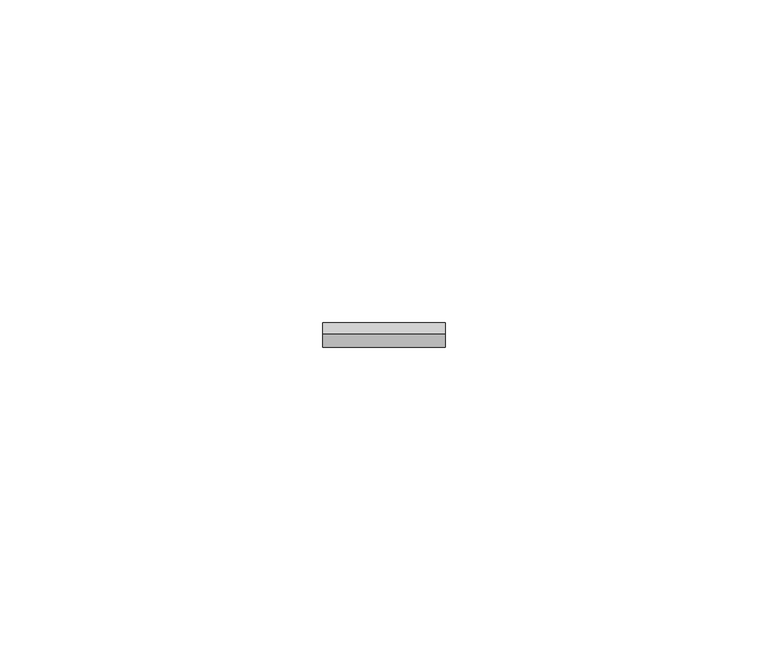
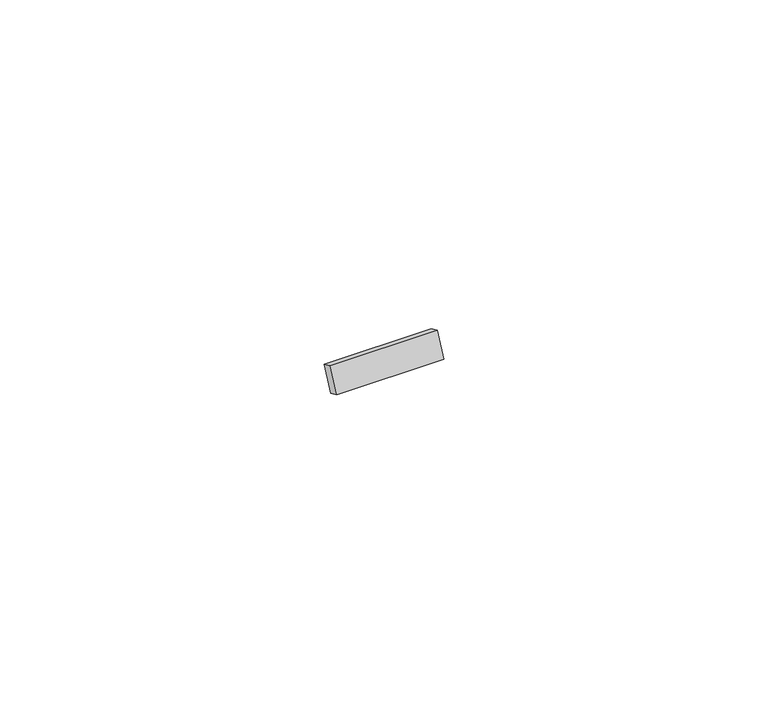
"""IFC4 building model written with IfcOpenShell, lengths in millimetres: furniture geometry, MOLDURA TELA1 : MOLDURA TELA."""

from ifc_helpers import new_model, si_unit, frame, origin, place, context, project, spatial, polyline, outline, extrude, source, transform, mapped, element, save


def furniture_bc1ec6cb(model_context):
    return source(origin(), model_context, "Body", "SweptSolid", [
        extrude(outline(polyline([(0.0, -19.0), (0.0, 0.0), (2.0, 0.0), (2.0, -19.0), (0.0, -19.0)])), frame((2400.0719295, 1317.2941444, 58.8666666), z_axis=(0.0, 0.4226182617406868, 0.9063077870366559), x_axis=(0.0, -0.9063077870366559, 0.4226182617406868)), (0.0, 0.0, 1.0), 4.7),
    ])


if __name__ == "__main__":
    model = new_model("IFC4")
    model_context = context("Model", 3, world=origin())
    ifc_project = project(units=[si_unit("LENGTHUNIT", "METRE", prefix="MILLI")], contexts=[model_context])
    site = spatial("IfcSite", under=ifc_project)
    building = spatial("IfcBuilding", under=site)
    placement = place(None, origin())
    furniture_shape = furniture_bc1ec6cb(model_context)
    element("IfcFurniture", 1, ObjectType="MOLDURA TELA1 : MOLDURA TELA", at=placement, inside=building, context=model_context, shape_type="MappedRepresentation", body=[
        mapped(furniture_shape, transform((0.0, 0.0, 0.0), x_axis=(1.0, 0.0, 0.0), y_axis=(0.0, 1.0, 0.0), z_axis=(0.0, 0.0, 1.0))),
    ])
    save(model, "model.ifc")

# Revit data of these elements
# Type "MOLDURA TELA1 : MOLDURA TELA"
#   Height = 0
# Element 1 (IfcFurniture, "MOLDURA TELA1 : MOLDURA TELA")
#   Materials on its faces: ".BOX FUNDO"
# Materials
#   ".BOX FUNDO": class "Vidro", colour RGB 236 240 239, transparency 0.15, Cost = 0
